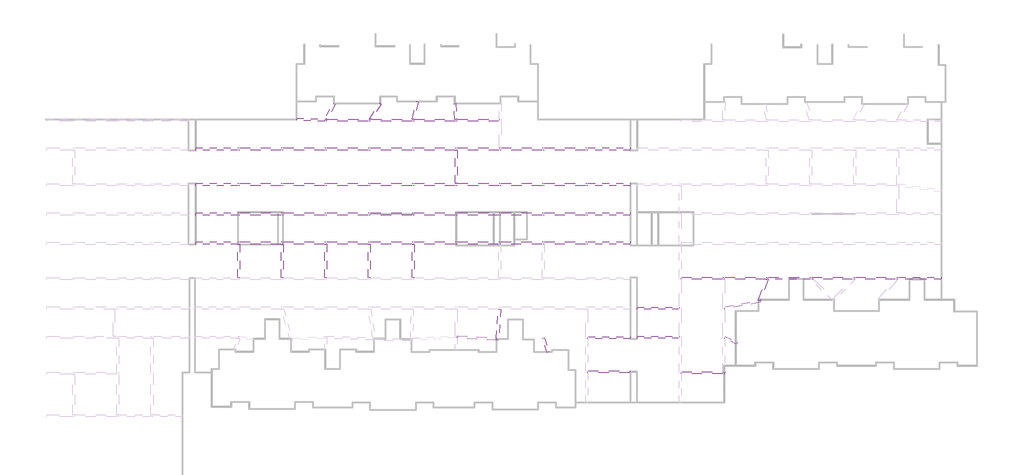
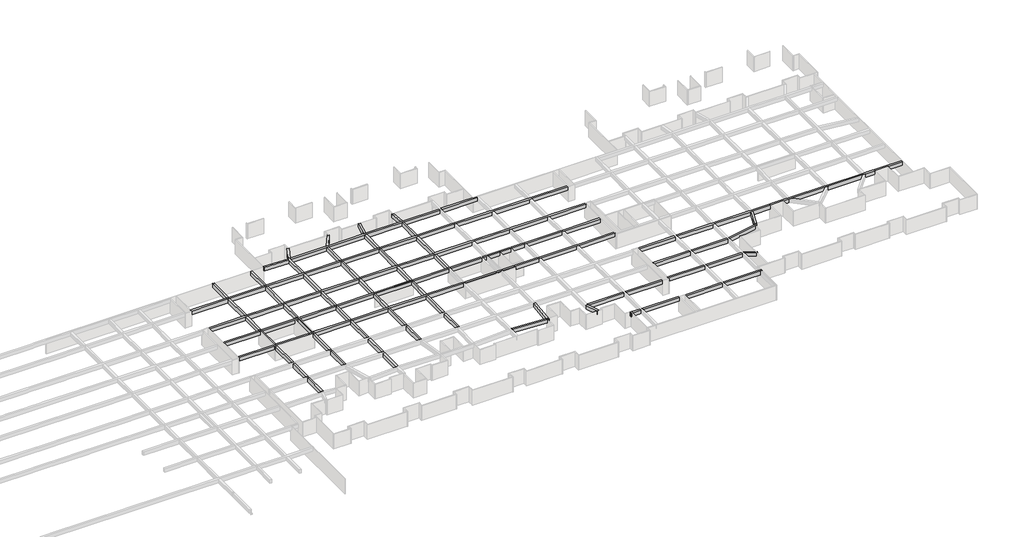
# One storey, part 15 of 16: 28 beams.
"""IFC4 building model written with IfcOpenShell, lengths in millimetres."""

from ifc_helpers import new_model, si_unit, frame, origin, place, context, project, spatial, polyline, outline, extrude, faceted_brep, element, save

model = new_model("IFC4")

# Units and contexts
model_context = context("Model", 3, world=origin())
ifc_project = project(units=[si_unit("LENGTHUNIT", "METRE", prefix="MILLI")], contexts=[model_context])

# Site, building, storey
site = spatial("IfcSite", under=ifc_project)
building = spatial("IfcBuilding", under=site)
storey = spatial("IfcBuildingStorey", under=building, Name="户型图", Elevation=0.0)

# Beams
placement = place(None, origin())
element("IfcBeam", 1, ObjectType="混凝土 - 矩形梁 : KL_beam", at=placement, inside=storey, context=model_context, shape_type="Brep", body=[
    faceted_brep([(413278.7576761, -137565.7214763, 3300.0), (413278.7576761, -137965.7214763, 3300.0), (413278.7576761, -137965.7214763, 2500.0), (413278.7576761, -137565.7214763, 2500.0), (333303.7576761, -137565.7214763, 3300.0), (333303.7576761, -137565.7214763, 2500.0), (333303.7576761, -137965.7214763, 2500.0), (333303.7576761, -137965.7214763, 3300.0), (405478.7576761, -137565.7214763, 3300.0), (405078.7576761, -137565.7214763, 3300.0), (397425.7298502, -137565.7214763, 3300.0), (397025.7298502, -137565.7214763, 3300.0), (389513.757676, -137565.7214763, 3300.0), (389113.757676, -137565.7214763, 3300.0), (381435.9353884, -137565.7214763, 3300.0), (381035.9353884, -137565.7214763, 3300.0), (373507.5350349, -137565.7214763, 3300.0), (373107.5350349, -137565.7214763, 3300.0), (365445.2144882, -137565.7214763, 3300.0), (365045.2144882, -137565.7214763, 3300.0), (357429.5901603, -137565.7214763, 3300.0), (357029.5901603, -137565.7214763, 3300.0), (349446.5285699, -137565.7214763, 3300.0), (349046.5285699, -137565.7214763, 3300.0), (341453.7576761, -137565.7214763, 3300.0), (341053.7576761, -137565.7214763, 3300.0), (341053.7576761, -137965.7214763, 3300.0), (341453.7576761, -137965.7214763, 3300.0), (349046.5285699, -137965.7214763, 3300.0), (349446.5285699, -137965.7214763, 3300.0), (357029.5901603, -137965.7214763, 3300.0), (357429.5901603, -137965.7214763, 3300.0), (365045.2144882, -137965.7214763, 3300.0), (365445.2144882, -137965.7214763, 3300.0), (373107.5350349, -137965.7214763, 3300.0), (373507.5350349, -137965.7214763, 3300.0), (381035.9353884, -137965.7214763, 3300.0), (381435.9353884, -137965.7214763, 3300.0), (389113.757676, -137965.7214763, 3300.0), (389513.757676, -137965.7214763, 3300.0), (397025.7298502, -137965.7214763, 3300.0), (397425.7298502, -137965.7214763, 3300.0), (405078.7576761, -137965.7214763, 3300.0), (405478.7576761, -137965.7214763, 3300.0), (341053.7576761, -137965.7214763, 2500.0), (341453.7576761, -137965.7214763, 2500.0), (349046.5285699, -137965.7214763, 2500.0), (349446.5285699, -137965.7214763, 2500.0), (357029.5901603, -137965.7214763, 2500.0), (357429.5901603, -137965.7214763, 2500.0), (365045.2144882, -137965.7214763, 2500.0), (365445.2144882, -137965.7214763, 2500.0), (373107.5350349, -137965.7214763, 2500.0), (373507.5350349, -137965.7214763, 2500.0), (381035.9353884, -137965.7214763, 2500.0), (381435.9353884, -137965.7214763, 2500.0), (389113.757676, -137965.7214763, 2500.0), (389513.757676, -137965.7214763, 2500.0), (397025.7298502, -137965.7214763, 2500.0), (397425.7298502, -137965.7214763, 2500.0), (405078.7576761, -137965.7214763, 2500.0), (405478.7576761, -137965.7214763, 2500.0), (341053.7576761, -137565.7214763, 2500.0), (341453.7576761, -137565.7214763, 2500.0), (349046.5285699, -137565.7214763, 2500.0), (349446.5285699, -137565.7214763, 2500.0), (357029.5901603, -137565.7214763, 2500.0), (357429.5901603, -137565.7214763, 2500.0), (365045.2144882, -137565.7214763, 2500.0), (365445.2144882, -137565.7214763, 2500.0), (373107.5350349, -137565.7214763, 2500.0), (373507.5350349, -137565.7214763, 2500.0), (381035.9353884, -137565.7214763, 2500.0), (381435.9353884, -137565.7214763, 2500.0), (389113.757676, -137565.7214763, 2500.0), (389513.757676, -137565.7214763, 2500.0), (397025.7298502, -137565.7214763, 2500.0), (397425.7298502, -137565.7214763, 2500.0), (405078.7576761, -137565.7214763, 2500.0), (405478.7576761, -137565.7214763, 2500.0)], [[[0, 1, 2, 3]], [[4, 5, 6, 7]], [[1, 0, 8, 9, 10, 11, 12, 13, 14, 15, 16, 17, 18, 19, 20, 21, 22, 23, 24, 25, 4, 7, 26, 27, 28, 29, 30, 31, 32, 33, 34, 35, 36, 37, 38, 39, 40, 41, 42, 43]], [[2, 1, 43, 42, 41, 40, 39, 38, 37, 36, 35, 34, 33, 32, 31, 30, 29, 28, 27, 26, 7, 6, 44, 45, 46, 47, 48, 49, 50, 51, 52, 53, 54, 55, 56, 57, 58, 59, 60, 61]], [[3, 2, 61, 60, 59, 58, 57, 56, 55, 54, 53, 52, 51, 50, 49, 48, 47, 46, 45, 44, 6, 5, 62, 63, 64, 65, 66, 67, 68, 69, 70, 71, 72, 73, 74, 75, 76, 77, 78, 79]], [[0, 3, 79, 78, 77, 76, 75, 74, 73, 72, 71, 70, 69, 68, 67, 66, 65, 64, 63, 62, 5, 4, 25, 24, 23, 22, 21, 20, 19, 18, 17, 16, 15, 14, 13, 12, 11, 10, 9, 8]]]),
])
element("IfcBeam", 2, ObjectType="混凝土 - 矩形梁 : KL_beam", at=placement, inside=storey, context=model_context, shape_type="Brep", body=[
    faceted_brep([(413278.7576761, -144085.7214763, 3300.0), (413278.7576761, -144485.7214763, 3300.0), (413278.7576761, -144485.7214763, 2500.0), (413278.7576761, -144085.7214763, 2500.0), (333303.7576761, -144085.7214763, 3300.0), (333303.7576761, -144085.7214763, 2500.0), (333303.7576761, -144485.7214763, 2500.0), (333303.7576761, -144485.7214763, 3300.0), (405478.7576761, -144085.7214763, 3300.0), (405078.7576761, -144085.7214763, 3300.0), (397425.7298502, -144085.7214763, 3300.0), (397025.7298502, -144085.7214763, 3300.0), (389513.757676, -144085.7214763, 3300.0), (389113.757676, -144085.7214763, 3300.0), (381435.9353884, -144085.7214763, 3300.0), (381035.9353884, -144085.7214763, 3300.0), (373507.5350349, -144085.7214763, 3300.0), (373107.5350349, -144085.7214763, 3300.0), (365445.2144882, -144085.7214763, 3300.0), (365045.2144882, -144085.7214763, 3300.0), (357429.5901603, -144085.7214763, 3300.0), (357029.5901603, -144085.7214763, 3300.0), (349446.5285699, -144085.7214763, 3300.0), (349046.5285699, -144085.7214763, 3300.0), (341453.7576761, -144085.7214763, 3300.0), (341053.7576761, -144085.7214763, 3300.0), (341053.7576761, -144485.7214763, 3300.0), (341453.7576761, -144485.7214763, 3300.0), (349046.5285699, -144485.7214763, 3300.0), (349446.5285699, -144485.7214763, 3300.0), (357029.5901603, -144485.7214763, 3300.0), (357429.5901603, -144485.7214763, 3300.0), (365045.2144882, -144485.7214763, 3300.0), (365445.2144882, -144485.7214763, 3300.0), (373107.5350349, -144485.7214763, 3300.0), (373507.5350349, -144485.7214763, 3300.0), (381035.9353884, -144485.7214763, 3300.0), (381435.9353884, -144485.7214763, 3300.0), (389113.757676, -144485.7214763, 3300.0), (389513.757676, -144485.7214763, 3300.0), (397025.7298502, -144485.7214763, 3300.0), (397425.7298502, -144485.7214763, 3300.0), (405078.7576761, -144485.7214763, 3300.0), (405478.7576761, -144485.7214763, 3300.0), (341053.7576761, -144485.7214763, 2500.0), (341453.7576761, -144485.7214763, 2500.0), (349046.5285699, -144485.7214763, 2500.0), (349446.5285699, -144485.7214763, 2500.0), (357029.5901603, -144485.7214763, 2500.0), (357429.5901603, -144485.7214763, 2500.0), (365045.2144882, -144485.7214763, 2500.0), (365445.2144882, -144485.7214763, 2500.0), (373107.5350349, -144485.7214763, 2500.0), (373507.5350349, -144485.7214763, 2500.0), (381035.9353884, -144485.7214763, 2500.0), (381435.9353884, -144485.7214763, 2500.0), (389113.757676, -144485.7214763, 2500.0), (389513.757676, -144485.7214763, 2500.0), (397025.7298502, -144485.7214763, 2500.0), (397425.7298502, -144485.7214763, 2500.0), (405078.7576761, -144485.7214763, 2500.0), (405478.7576761, -144485.7214763, 2500.0), (341053.7576761, -144085.7214763, 2500.0), (341453.7576761, -144085.7214763, 2500.0), (349046.5285699, -144085.7214763, 2500.0), (349446.5285699, -144085.7214763, 2500.0), (357029.5901603, -144085.7214763, 2500.0), (357429.5901603, -144085.7214763, 2500.0), (365045.2144882, -144085.7214763, 2500.0), (365445.2144882, -144085.7214763, 2500.0), (373107.5350349, -144085.7214763, 2500.0), (373507.5350349, -144085.7214763, 2500.0), (381035.9353884, -144085.7214763, 2500.0), (381435.9353884, -144085.7214763, 2500.0), (389113.757676, -144085.7214763, 2500.0), (389513.757676, -144085.7214763, 2500.0), (397025.7298502, -144085.7214763, 2500.0), (397425.7298502, -144085.7214763, 2500.0), (405078.7576761, -144085.7214763, 2500.0), (405478.7576761, -144085.7214763, 2500.0)], [[[0, 1, 2, 3]], [[4, 5, 6, 7]], [[1, 0, 8, 9, 10, 11, 12, 13, 14, 15, 16, 17, 18, 19, 20, 21, 22, 23, 24, 25, 4, 7, 26, 27, 28, 29, 30, 31, 32, 33, 34, 35, 36, 37, 38, 39, 40, 41, 42, 43]], [[2, 1, 43, 42, 41, 40, 39, 38, 37, 36, 35, 34, 33, 32, 31, 30, 29, 28, 27, 26, 7, 6, 44, 45, 46, 47, 48, 49, 50, 51, 52, 53, 54, 55, 56, 57, 58, 59, 60, 61]], [[3, 2, 61, 60, 59, 58, 57, 56, 55, 54, 53, 52, 51, 50, 49, 48, 47, 46, 45, 44, 6, 5, 62, 63, 64, 65, 66, 67, 68, 69, 70, 71, 72, 73, 74, 75, 76, 77, 78, 79]], [[0, 3, 79, 78, 77, 76, 75, 74, 73, 72, 71, 70, 69, 68, 67, 66, 65, 64, 63, 62, 5, 4, 25, 24, 23, 22, 21, 20, 19, 18, 17, 16, 15, 14, 13, 12, 11, 10, 9, 8]]]),
])
element("IfcBeam", 3, ObjectType="混凝土 - 矩形梁 : KL_beam", at=placement, inside=storey, context=model_context, shape_type="Brep", body=[
    faceted_brep([(413278.7576761, -149515.4343269, 3300.0), (413278.7576761, -149915.4343269, 3300.0), (413278.7576761, -149915.4343269, 2500.0), (413278.7576761, -149515.4343269, 2500.0), (333303.7576761, -149515.4343269, 3300.0), (333303.7576761, -149515.4343269, 2500.0), (333303.7576761, -149915.4343269, 2500.0), (333303.7576761, -149915.4343269, 3300.0), (405478.7576761, -149515.4343269, 3300.0), (405078.7576761, -149515.4343269, 3300.0), (397425.7298502, -149515.4343269, 3300.0), (397025.7298502, -149515.4343269, 3300.0), (389513.757676, -149515.4343269, 3300.0), (389113.757676, -149515.4343269, 3300.0), (381435.9353884, -149515.4343269, 3300.0), (381035.9353884, -149515.4343269, 3300.0), (373507.5350349, -149515.4343269, 3300.0), (373107.5350349, -149515.4343269, 3300.0), (365445.2144882, -149515.4343269, 3300.0), (365045.2144882, -149515.4343269, 3300.0), (357429.5901603, -149515.4343269, 3300.0), (357029.5901603, -149515.4343269, 3300.0), (349446.5285699, -149515.4343269, 3300.0), (349046.5285699, -149515.4343269, 3300.0), (341453.7576761, -149515.4343269, 3300.0), (341053.7576761, -149515.4343269, 3300.0), (341053.7576761, -149915.4343269, 3300.0), (341453.7576761, -149915.4343269, 3300.0), (349046.5285699, -149915.4343269, 3300.0), (349446.5285699, -149915.4343269, 3300.0), (357029.5901603, -149915.4343269, 3300.0), (357429.5901603, -149915.4343269, 3300.0), (365045.2144882, -149915.4343269, 3300.0), (365445.2144882, -149915.4343269, 3300.0), (373107.5350349, -149915.4343269, 3300.0), (373507.5350349, -149915.4343269, 3300.0), (381035.9353884, -149915.4343269, 3300.0), (381435.9353884, -149915.4343269, 3300.0), (389033.5747738, -149915.4343269, 3300.0), (389433.5747738, -149915.4343269, 3300.0), (397025.7298502, -149915.4343269, 3300.0), (397425.7298502, -149915.4343269, 3300.0), (405078.7576761, -149915.4343269, 3300.0), (405478.7576761, -149915.4343269, 3300.0), (341053.7576761, -149915.4343269, 2500.0), (341453.7576761, -149915.4343269, 2500.0), (349046.5285699, -149915.4343269, 2500.0), (349446.5285699, -149915.4343269, 2500.0), (357029.5901603, -149915.4343269, 2500.0), (357429.5901603, -149915.4343269, 2500.0), (365045.2144882, -149915.4343269, 2500.0), (365445.2144882, -149915.4343269, 2500.0), (373107.5350349, -149915.4343269, 2500.0), (373507.5350349, -149915.4343269, 2500.0), (381035.9353884, -149915.4343269, 2500.0), (381435.9353884, -149915.4343269, 2500.0), (389033.5747738, -149915.4343269, 2500.0), (389433.5747738, -149915.4343269, 2500.0), (397025.7298502, -149915.4343269, 2500.0), (397425.7298502, -149915.4343269, 2500.0), (405078.7576761, -149915.4343269, 2500.0), (405478.7576761, -149915.4343269, 2500.0), (341053.7576761, -149515.4343269, 2500.0), (341453.7576761, -149515.4343269, 2500.0), (349046.5285699, -149515.4343269, 2500.0), (349446.5285699, -149515.4343269, 2500.0), (357029.5901603, -149515.4343269, 2500.0), (357429.5901603, -149515.4343269, 2500.0), (365045.2144882, -149515.4343269, 2500.0), (365445.2144882, -149515.4343269, 2500.0), (373107.5350349, -149515.4343269, 2500.0), (373507.5350349, -149515.4343269, 2500.0), (381035.9353884, -149515.4343269, 2500.0), (381435.9353884, -149515.4343269, 2500.0), (389113.757676, -149515.4343269, 2500.0), (389513.757676, -149515.4343269, 2500.0), (397025.7298502, -149515.4343269, 2500.0), (397425.7298502, -149515.4343269, 2500.0), (405078.7576761, -149515.4343269, 2500.0), (405478.7576761, -149515.4343269, 2500.0)], [[[0, 1, 2, 3]], [[4, 5, 6, 7]], [[1, 0, 8, 9, 10, 11, 12, 13, 14, 15, 16, 17, 18, 19, 20, 21, 22, 23, 24, 25, 4, 7, 26, 27, 28, 29, 30, 31, 32, 33, 34, 35, 36, 37, 38, 39, 40, 41, 42, 43]], [[2, 1, 43, 42, 41, 40, 39, 38, 37, 36, 35, 34, 33, 32, 31, 30, 29, 28, 27, 26, 7, 6, 44, 45, 46, 47, 48, 49, 50, 51, 52, 53, 54, 55, 56, 57, 58, 59, 60, 61]], [[3, 2, 61, 60, 59, 58, 57, 56, 55, 54, 53, 52, 51, 50, 49, 48, 47, 46, 45, 44, 6, 5, 62, 63, 64, 65, 66, 67, 68, 69, 70, 71, 72, 73, 74, 75, 76, 77, 78, 79]], [[0, 3, 79, 78, 77, 76, 75, 74, 73, 72, 71, 70, 69, 68, 67, 66, 65, 64, 63, 62, 5, 4, 25, 24, 23, 22, 21, 20, 19, 18, 17, 16, 15, 14, 13, 12, 11, 10, 9, 8]]]),
])
element("IfcBeam", 4, ObjectType="混凝土 - 矩形梁 : KL_beam", at=placement, inside=storey, context=model_context, shape_type="Brep", body=[
    faceted_brep([(413278.7576761, -154845.1471774, 3300.0), (413278.7576761, -155245.1471774, 3300.0), (413278.7576761, -155245.1471774, 2500.0), (413278.7576761, -154845.1471774, 2500.0), (333303.7576761, -154845.1471774, 3300.0), (333303.7576761, -154845.1471774, 2500.0), (333303.7576761, -155245.1471774, 2500.0), (333303.7576761, -155245.1471774, 3300.0), (405478.7576761, -154845.1471774, 3300.0), (405078.7576761, -154845.1471774, 3300.0), (397425.7298502, -154845.1471774, 3300.0), (397025.7298502, -154845.1471774, 3300.0), (389433.5747738, -154845.1471774, 3300.0), (389033.5747738, -154845.1471774, 3300.0), (381435.9353884, -154845.1471774, 3300.0), (381035.9353884, -154845.1471774, 3300.0), (373507.5350349, -154845.1471774, 3300.0), (373107.5350349, -154845.1471774, 3300.0), (365445.2144882, -154845.1471774, 3300.0), (365045.2144882, -154845.1471774, 3300.0), (357429.5901603, -154845.1471774, 3300.0), (357029.5901603, -154845.1471774, 3300.0), (349446.5285699, -154845.1471774, 3300.0), (349046.5285699, -154845.1471774, 3300.0), (341453.7576761, -154845.1471774, 3300.0), (341053.7576761, -154845.1471774, 3300.0), (341053.7576761, -155245.1471774, 3300.0), (341453.7576761, -155245.1471774, 3300.0), (349046.5285699, -155245.1471774, 3300.0), (349446.5285699, -155245.1471774, 3300.0), (357029.5901603, -155245.1471774, 3300.0), (357429.5901603, -155245.1471774, 3300.0), (365045.2144882, -155245.1471774, 3300.0), (365445.2144882, -155245.1471774, 3300.0), (373107.5350349, -155245.1471774, 3300.0), (373507.5350349, -155245.1471774, 3300.0), (381035.9353884, -155245.1471774, 3300.0), (381435.9353884, -155245.1471774, 3300.0), (389033.5747738, -155245.1471774, 3300.0), (389433.5747738, -155245.1471774, 3300.0), (397025.7298502, -155245.1471774, 3300.0), (397425.7298502, -155245.1471774, 3300.0), (405078.7576761, -155245.1471774, 3300.0), (405478.7576761, -155245.1471774, 3300.0), (341053.7576761, -155245.1471774, 2500.0), (341453.7576761, -155245.1471774, 2500.0), (349046.5285699, -155245.1471774, 2500.0), (349446.5285699, -155245.1471774, 2500.0), (357029.5901603, -155245.1471774, 2500.0), (357429.5901603, -155245.1471774, 2500.0), (365045.2144882, -155245.1471774, 2500.0), (365445.2144882, -155245.1471774, 2500.0), (373107.5350349, -155245.1471774, 2500.0), (373507.5350349, -155245.1471774, 2500.0), (381035.9353884, -155245.1471774, 2500.0), (381435.9353884, -155245.1471774, 2500.0), (389033.5747738, -155245.1471774, 2500.0), (389433.5747738, -155245.1471774, 2500.0), (397025.7298502, -155245.1471774, 2500.0), (397425.7298502, -155245.1471774, 2500.0), (405078.7576761, -155245.1471774, 2500.0), (405478.7576761, -155245.1471774, 2500.0), (341053.7576761, -154845.1471774, 2500.0), (341453.7576761, -154845.1471774, 2500.0), (349046.5285699, -154845.1471774, 2500.0), (349446.5285699, -154845.1471774, 2500.0), (357029.5901603, -154845.1471774, 2500.0), (357429.5901603, -154845.1471774, 2500.0), (365045.2144882, -154845.1471774, 2500.0), (365445.2144882, -154845.1471774, 2500.0), (373107.5350349, -154845.1471774, 2500.0), (373507.5350349, -154845.1471774, 2500.0), (381035.9353884, -154845.1471774, 2500.0), (381435.9353884, -154845.1471774, 2500.0), (389033.5747738, -154845.1471774, 2500.0), (389433.5747738, -154845.1471774, 2500.0), (397025.7298502, -154845.1471774, 2500.0), (397425.7298502, -154845.1471774, 2500.0), (405078.7576761, -154845.1471774, 2500.0), (405478.7576761, -154845.1471774, 2500.0)], [[[0, 1, 2, 3]], [[4, 5, 6, 7]], [[1, 0, 8, 9, 10, 11, 12, 13, 14, 15, 16, 17, 18, 19, 20, 21, 22, 23, 24, 25, 4, 7, 26, 27, 28, 29, 30, 31, 32, 33, 34, 35, 36, 37, 38, 39, 40, 41, 42, 43]], [[2, 1, 43, 42, 41, 40, 39, 38, 37, 36, 35, 34, 33, 32, 31, 30, 29, 28, 27, 26, 7, 6, 44, 45, 46, 47, 48, 49, 50, 51, 52, 53, 54, 55, 56, 57, 58, 59, 60, 61]], [[3, 2, 61, 60, 59, 58, 57, 56, 55, 54, 53, 52, 51, 50, 49, 48, 47, 46, 45, 44, 6, 5, 62, 63, 64, 65, 66, 67, 68, 69, 70, 71, 72, 73, 74, 75, 76, 77, 78, 79]], [[0, 3, 79, 78, 77, 76, 75, 74, 73, 72, 71, 70, 69, 68, 67, 66, 65, 64, 63, 62, 5, 4, 25, 24, 23, 22, 21, 20, 19, 18, 17, 16, 15, 14, 13, 12, 11, 10, 9, 8]]]),
])
element("IfcBeam", 5, ObjectType="混凝土 - 矩形梁 : KL_beam", at=placement, inside=storey, context=model_context, shape_type="Brep", body=[
    faceted_brep([(341053.7576761, -132205.3490877, 3300.0), (341453.7576761, -132205.3490877, 3300.0), (341453.7576761, -132205.3490877, 2500.0), (341053.7576761, -132205.3490877, 2500.0), (341053.7576761, -137565.7214763, 3300.0), (341453.7576761, -137565.7214763, 3300.0), (341453.7576761, -137565.7214763, 2500.0), (341053.7576761, -137565.7214763, 2500.0)], [[[0, 1, 2, 3]], [[1, 0, 4, 5]], [[2, 1, 5, 6]], [[3, 2, 6, 7]], [[0, 3, 7, 4]], [[5, 4, 7, 6]]]),
    faceted_brep([(341053.7576761, -172220.550998, 3300.0), (341053.7576761, -172220.550998, 2500.0), (341105.8656487, -172220.550998, 2500.0), (341263.4411641, -172220.550998, 2500.0), (341263.4411641, -172220.550998, 3300.0), (341105.8656487, -172220.550998, 3300.0), (341453.7576761, -172239.0235791, 3300.0), (341453.7576761, -172239.0235791, 2500.0), (341053.7576761, -167205.1471774, 3300.0), (341453.7576761, -167205.1471774, 3300.0), (341453.7576761, -167205.1471774, 2500.0), (341053.7576761, -167205.1471774, 2500.0)], [[[0, 1, 2, 3, 4, 5]], [[6, 4, 3, 7]], [[8, 9, 10, 11]], [[4, 6, 9, 8, 0, 5]], [[6, 7, 10, 9]], [[7, 3, 2, 1, 11, 10]], [[1, 0, 8, 11]]]),
    faceted_brep([(341053.7576761, -137965.7214763, 3300.0), (341453.7576761, -137965.7214763, 3300.0), (341453.7576761, -137965.7214763, 2500.0), (341053.7576761, -137965.7214763, 2500.0), (341053.7576761, -144085.7214763, 3300.0), (341453.7576761, -144085.7214763, 3300.0), (341453.7576761, -144085.7214763, 2500.0), (341053.7576761, -144085.7214763, 2500.0)], [[[0, 1, 2, 3]], [[1, 0, 4, 5]], [[2, 1, 5, 6]], [[3, 2, 6, 7]], [[0, 3, 7, 4]], [[5, 4, 7, 6]]]),
    faceted_brep([(341053.7576761, -144485.7214763, 3300.0), (341453.7576761, -144485.7214763, 3300.0), (341453.7576761, -144485.7214763, 2500.0), (341053.7576761, -144485.7214763, 2500.0), (341053.7576761, -149515.4343269, 3300.0), (341453.7576761, -149515.4343269, 3300.0), (341453.7576761, -149515.4343269, 2500.0), (341053.7576761, -149515.4343269, 2500.0)], [[[0, 1, 2, 3]], [[1, 0, 4, 5]], [[2, 1, 5, 6]], [[3, 2, 6, 7]], [[0, 3, 7, 4]], [[5, 4, 7, 6]]]),
    faceted_brep([(341053.7576761, -149915.4343269, 3300.0), (341453.7576761, -149915.4343269, 3300.0), (341453.7576761, -149915.4343269, 2500.0), (341053.7576761, -149915.4343269, 2500.0), (341053.7576761, -154845.1471774, 3300.0), (341453.7576761, -154845.1471774, 3300.0), (341453.7576761, -154845.1471774, 2500.0), (341053.7576761, -154845.1471774, 2500.0)], [[[0, 1, 2, 3]], [[1, 0, 4, 5]], [[2, 1, 5, 6]], [[3, 2, 6, 7]], [[0, 3, 7, 4]], [[5, 4, 7, 6]]]),
    faceted_brep([(341053.7576761, -155245.1471774, 3300.0), (341453.7576761, -155245.1471774, 3300.0), (341453.7576761, -155245.1471774, 2500.0), (341053.7576761, -155245.1471774, 2500.0), (341053.7576761, -161426.0461868, 3300.0), (341453.7576761, -161426.0461868, 3300.0), (341453.7576761, -161426.0461868, 2500.0), (341053.7576761, -161426.0461868, 2500.0)], [[[0, 1, 2, 3]], [[1, 0, 4, 5]], [[2, 1, 5, 6]], [[3, 2, 6, 7]], [[0, 3, 7, 4]], [[5, 4, 7, 6]]]),
    faceted_brep([(341053.7576761, -161826.0461868, 3300.0), (341453.7576761, -161826.0461868, 3300.0), (341453.7576761, -161826.0461868, 2500.0), (341053.7576761, -161826.0461868, 2500.0), (341053.7576761, -166805.1471774, 3300.0), (341453.7576761, -166805.1471774, 3300.0), (341453.7576761, -166805.1471774, 2500.0), (341053.7576761, -166805.1471774, 2500.0)], [[[0, 1, 2, 3]], [[1, 0, 4, 5]], [[2, 1, 5, 6]], [[3, 2, 6, 7]], [[0, 3, 7, 4]], [[5, 4, 7, 6]]]),
])
element("IfcBeam", 6, ObjectType="混凝土 - 矩形梁 : KL_beam", at=placement, inside=storey, context=model_context, shape_type="SweptSolid", body=[
    extrude(outline(polyline([(349046.5285699, -132305.1471774), (349446.5285699, -132305.1471774), (349446.5285699, -137565.7214763), (349046.5285699, -137565.7214763), (349046.5285699, -132305.1471774)])), frame((0.0, 0.0, 2500.0), z_axis=(0.0, 0.0, 1.0), x_axis=(1.0, 0.0, 0.0)), (0.0, 0.0, 1.0), 800.0),
    extrude(outline(polyline([(349046.5285699, -137965.7214763), (349446.5285699, -137965.7214763), (349446.5285699, -144085.7214763), (349046.5285699, -144085.7214763), (349046.5285699, -137965.7214763)])), frame((0.0, 0.0, 2500.0), z_axis=(0.0, 0.0, 1.0), x_axis=(1.0, 0.0, 0.0)), (0.0, 0.0, 1.0), 800.0),
    extrude(outline(polyline([(349446.5285699, -166805.1471774), (349046.5285699, -166805.1471774), (349046.5285699, -161826.0461868), (349446.5285699, -161826.0461868), (349446.5285699, -166805.1471774)])), frame((0.0, 0.0, 2500.0), z_axis=(0.0, 0.0, 1.0), x_axis=(1.0, 0.0, 0.0)), (0.0, 0.0, 1.0), 800.0),
    extrude(outline(polyline([(349046.5285699, -144485.7214763), (349446.5285699, -144485.7214763), (349446.5285699, -149515.4343269), (349046.5285699, -149515.4343269), (349046.5285699, -144485.7214763)])), frame((0.0, 0.0, 2500.0), z_axis=(0.0, 0.0, 1.0), x_axis=(1.0, 0.0, 0.0)), (0.0, 0.0, 1.0), 800.0),
    extrude(outline(polyline([(349046.5285699, -149915.4343269), (349446.5285699, -149915.4343269), (349446.5285699, -154845.1471774), (349046.5285699, -154845.1471774), (349046.5285699, -149915.4343269)])), frame((0.0, 0.0, 2500.0), z_axis=(0.0, 0.0, 1.0), x_axis=(1.0, 0.0, 0.0)), (0.0, 0.0, 1.0), 800.0),
    extrude(outline(polyline([(349046.5285699, -155245.1471774), (349446.5285699, -155245.1471774), (349446.5285699, -161426.0461868), (349046.5285699, -161426.0461868), (349046.5285699, -155245.1471774)])), frame((0.0, 0.0, 2500.0), z_axis=(0.0, 0.0, 1.0), x_axis=(1.0, 0.0, 0.0)), (0.0, 0.0, 1.0), 800.0),
])
element("IfcBeam", 7, ObjectType="混凝土 - 矩形梁 : KL_beam", at=placement, inside=storey, context=model_context, shape_type="Brep", body=[
    faceted_brep([(357029.5901603, -137565.7214763, 3300.0), (357429.5901603, -137565.7214763, 3300.0), (357429.5901603, -132682.1518701, 3300.0), (357429.5901603, -132528.9518593, 3300.0), (357429.5901603, -131627.4508185, 3300.0), (357107.4901686, -132278.0131322, 3300.0), (357029.5901603, -132435.3518808, 3300.0), (357029.5901603, -132675.6598872, 3300.0), (357429.5901603, -137565.7214763, 2500.0), (357429.5901603, -132682.1518701, 2500.0), (357429.5901603, -132528.9518593, 2500.0), (357429.5901603, -131627.4508185, 2500.0), (357029.5901603, -137565.7214763, 2500.0), (357029.5901603, -132675.6598872, 2500.0), (357029.5901603, -132435.3518808, 2500.0), (357107.4901686, -132278.0131322, 2500.0)], [[[0, 1, 2, 3, 4, 5, 6, 7]], [[1, 8, 9, 10, 11, 4, 3, 2]], [[8, 12, 13, 14, 15, 11, 10, 9]], [[12, 0, 7, 6, 14, 13]], [[1, 0, 12, 8]], [[6, 5, 4, 11, 15, 14]]]),
    faceted_brep([(357029.5901603, -137965.7214763, 3300.0), (357429.5901603, -137965.7214763, 3300.0), (357429.5901603, -137965.7214763, 2500.0), (357029.5901603, -137965.7214763, 2500.0), (357029.5901603, -144085.7214763, 3300.0), (357429.5901603, -144085.7214763, 3300.0), (357429.5901603, -144085.7214763, 2500.0), (357029.5901603, -144085.7214763, 2500.0)], [[[0, 1, 2, 3]], [[1, 0, 4, 5]], [[2, 1, 5, 6]], [[3, 2, 6, 7]], [[0, 3, 7, 4]], [[5, 4, 7, 6]]]),
    faceted_brep([(357029.5901603, -144485.7214763, 3300.0), (357429.5901603, -144485.7214763, 3300.0), (357429.5901603, -144485.7214763, 2500.0), (357029.5901603, -144485.7214763, 2500.0), (357029.5901603, -149515.4343269, 3300.0), (357429.5901603, -149515.4343269, 3300.0), (357429.5901603, -149515.4343269, 2500.0), (357029.5901603, -149515.4343269, 2500.0)], [[[0, 1, 2, 3]], [[1, 0, 4, 5]], [[2, 1, 5, 6]], [[3, 2, 6, 7]], [[0, 3, 7, 4]], [[5, 4, 7, 6]]]),
    faceted_brep([(357029.5901603, -149915.4343269, 3300.0), (357429.5901603, -149915.4343269, 3300.0), (357429.5901603, -149915.4343269, 2500.0), (357029.5901603, -149915.4343269, 2500.0), (357029.5901603, -154845.1471774, 3300.0), (357429.5901603, -154845.1471774, 3300.0), (357429.5901603, -154845.1471774, 2500.0), (357029.5901603, -154845.1471774, 2500.0)], [[[0, 1, 2, 3]], [[1, 0, 4, 5]], [[2, 1, 5, 6]], [[3, 2, 6, 7]], [[0, 3, 7, 4]], [[5, 4, 7, 6]]]),
    faceted_brep([(357029.5901603, -155245.1471774, 3300.0), (357429.5901603, -155245.1471774, 3300.0), (357429.5901603, -155245.1471774, 2500.0), (357029.5901603, -155245.1471774, 2500.0), (357029.5901603, -161426.0461868, 3300.0), (357429.5901603, -161426.0461868, 3300.0), (357429.5901603, -161426.0461868, 2500.0), (357029.5901603, -161426.0461868, 2500.0)], [[[0, 1, 2, 3]], [[1, 0, 4, 5]], [[2, 1, 5, 6]], [[3, 2, 6, 7]], [[0, 3, 7, 4]], [[5, 4, 7, 6]]]),
    faceted_brep([(357029.5901603, -161826.0461868, 3300.0), (357429.5901603, -161826.0461868, 3300.0), (357429.5901603, -161826.0461868, 2500.0), (357029.5901603, -161826.0461868, 2500.0), (357029.5901603, -166805.1471774, 3300.0), (357429.5901603, -166805.1471774, 3300.0), (357429.5901603, -166805.1471774, 2500.0), (357029.5901603, -166805.1471774, 2500.0)], [[[0, 1, 2, 3]], [[1, 0, 4, 5]], [[2, 1, 5, 6]], [[3, 2, 6, 7]], [[0, 3, 7, 4]], [[5, 4, 7, 6]]]),
    faceted_brep([(357029.5901603, -167205.1471774, 3300.0), (357429.5901603, -167205.1471774, 3300.0), (357429.5901603, -167205.1471774, 2500.0), (357029.5901603, -167205.1471774, 2500.0), (357029.5901603, -172194.5475715, 3300.0), (357429.5901603, -172168.9371393, 3300.0), (357429.5901603, -172168.9371393, 2500.0), (357029.5901603, -172194.5475715, 2500.0)], [[[0, 1, 2, 3]], [[1, 0, 4, 5]], [[2, 1, 5, 6]], [[3, 2, 6, 7]], [[0, 3, 7, 4]], [[5, 4, 7, 6]]]),
])
element("IfcBeam", 8, ObjectType="混凝土 - 矩形梁 : KL_beam", at=placement, inside=storey, context=model_context, shape_type="Brep", body=[
    faceted_brep([(358578.5409484, -129306.8544128, 3300.0), (358937.0102239, -129484.3361824, 3300.0), (358937.0102239, -129484.3361824, 2500.0), (358578.5409484, -129306.8544128, 2500.0), (357429.5901603, -131627.4508185, 3300.0), (357429.5901603, -132528.9518593, 3300.0), (357551.7833351, -132282.1518701, 3300.0), (357429.5901603, -132528.9518593, 2500.0), (357551.7833351, -132282.1518701, 2500.0), (357429.5901603, -131627.4508185, 2500.0)], [[[0, 1, 2, 3]], [[1, 0, 4, 5, 6]], [[2, 1, 6, 5, 7, 8]], [[3, 2, 8, 7, 9]], [[0, 3, 9, 4]], [[5, 4, 9, 7]]]),
])
element("IfcBeam", 9, ObjectType="混凝土 - 矩形梁 : KL_beam", at=placement, inside=storey, context=model_context, shape_type="SweptSolid", body=[
    extrude(outline(polyline([(367089.0963461, -129289.7981648), (367428.3155846, -129501.7658705), (365690.937587, -132282.1518701), (365219.2662256, -132282.1518701), (367089.0963461, -129289.7981648)])), frame((0.0, 0.0, 2500.0), z_axis=(0.0, 0.0, 1.0), x_axis=(1.0, 0.0, 0.0)), (0.0, 0.0, 1.0), 800.0),
])
element("IfcBeam", 10, ObjectType="混凝土 - 矩形梁 : KL_beam", at=placement, inside=storey, context=model_context, shape_type="SweptSolid", body=[
    extrude(outline(polyline([(365045.2144882, -132682.1518701), (365445.2144882, -132682.1518701), (365445.2144882, -137565.7214763), (365045.2144882, -137565.7214763), (365045.2144882, -132682.1518701)])), frame((0.0, 0.0, 2500.0), z_axis=(0.0, 0.0, 1.0), x_axis=(1.0, 0.0, 0.0)), (0.0, 0.0, 1.0), 800.0),
    extrude(outline(polyline([(365445.2144882, -166805.1471774), (365045.2144882, -166805.1471774), (365045.2144882, -161826.0461868), (365445.2144882, -161826.0461868), (365445.2144882, -166805.1471774)])), frame((0.0, 0.0, 2500.0), z_axis=(0.0, 0.0, 1.0), x_axis=(1.0, 0.0, 0.0)), (0.0, 0.0, 1.0), 800.0),
    extrude(outline(polyline([(365045.2144882, -137965.7214763), (365445.2144882, -137965.7214763), (365445.2144882, -144085.7214763), (365045.2144882, -144085.7214763), (365045.2144882, -137965.7214763)])), frame((0.0, 0.0, 2500.0), z_axis=(0.0, 0.0, 1.0), x_axis=(1.0, 0.0, 0.0)), (0.0, 0.0, 1.0), 800.0),
    extrude(outline(polyline([(365045.2144882, -144485.7214763), (365445.2144882, -144485.7214763), (365445.2144882, -149515.4343269), (365045.2144882, -149515.4343269), (365045.2144882, -144485.7214763)])), frame((0.0, 0.0, 2500.0), z_axis=(0.0, 0.0, 1.0), x_axis=(1.0, 0.0, 0.0)), (0.0, 0.0, 1.0), 800.0),
    extrude(outline(polyline([(365045.2144882, -149915.4343269), (365445.2144882, -149915.4343269), (365445.2144882, -154845.1471774), (365045.2144882, -154845.1471774), (365045.2144882, -149915.4343269)])), frame((0.0, 0.0, 2500.0), z_axis=(0.0, 0.0, 1.0), x_axis=(1.0, 0.0, 0.0)), (0.0, 0.0, 1.0), 800.0),
    extrude(outline(polyline([(365045.2144882, -155245.1471774), (365445.2144882, -155245.1471774), (365445.2144882, -161426.0461868), (365045.2144882, -161426.0461868), (365045.2144882, -155245.1471774)])), frame((0.0, 0.0, 2500.0), z_axis=(0.0, 0.0, 1.0), x_axis=(1.0, 0.0, 0.0)), (0.0, 0.0, 1.0), 800.0),
])
element("IfcBeam", 11, ObjectType="混凝土 - 矩形梁 : KL_beam", at=placement, inside=storey, context=model_context, shape_type="SweptSolid", body=[
    extrude(outline(polyline([(373507.5350349, -166805.1471774), (373107.5350349, -166805.1471774), (373107.5350349, -161826.0461868), (373507.5350349, -161826.0461868), (373507.5350349, -166805.1471774)])), frame((0.0, 0.0, 2500.0), z_axis=(0.0, 0.0, 1.0), x_axis=(1.0, 0.0, 0.0)), (0.0, 0.0, 1.0), 800.0),
    extrude(outline(polyline([(373107.5350349, -137965.7214763), (373507.5350349, -137965.7214763), (373507.5350349, -144085.7214763), (373107.5350349, -144085.7214763), (373107.5350349, -137965.7214763)])), frame((0.0, 0.0, 2500.0), z_axis=(0.0, 0.0, 1.0), x_axis=(1.0, 0.0, 0.0)), (0.0, 0.0, 1.0), 800.0),
    extrude(outline(polyline([(373507.5350349, -137565.7214763), (373107.5350349, -137565.7214763), (373107.5350349, -132682.1518701), (373507.5350349, -132682.1518701), (373507.5350349, -137565.7214763)])), frame((0.0, 0.0, 2500.0), z_axis=(0.0, 0.0, 1.0), x_axis=(1.0, 0.0, 0.0)), (0.0, 0.0, 1.0), 800.0),
    extrude(outline(polyline([(373107.5350349, -144485.7214763), (373507.5350349, -144485.7214763), (373507.5350349, -149515.4343269), (373107.5350349, -149515.4343269), (373107.5350349, -144485.7214763)])), frame((0.0, 0.0, 2500.0), z_axis=(0.0, 0.0, 1.0), x_axis=(1.0, 0.0, 0.0)), (0.0, 0.0, 1.0), 800.0),
    extrude(outline(polyline([(373107.5350349, -149915.4343269), (373507.5350349, -149915.4343269), (373507.5350349, -154845.1471774), (373107.5350349, -154845.1471774), (373107.5350349, -149915.4343269)])), frame((0.0, 0.0, 2500.0), z_axis=(0.0, 0.0, 1.0), x_axis=(1.0, 0.0, 0.0)), (0.0, 0.0, 1.0), 800.0),
    extrude(outline(polyline([(373107.5350349, -155245.1471774), (373507.5350349, -155245.1471774), (373507.5350349, -161426.0461868), (373107.5350349, -161426.0461868), (373107.5350349, -155245.1471774)])), frame((0.0, 0.0, 2500.0), z_axis=(0.0, 0.0, 1.0), x_axis=(1.0, 0.0, 0.0)), (0.0, 0.0, 1.0), 800.0),
])
element("IfcBeam", 12, ObjectType="混凝土 - 矩形梁 : KL_beam", at=placement, inside=storey, context=model_context, shape_type="SweptSolid", body=[
    extrude(outline(polyline([(373860.3365631, -128942.4735942), (374251.5956034, -129025.6382705), (373559.4022696, -132282.1518701), (373150.4660317, -132282.1518701), (373860.3365631, -128942.4735942)])), frame((0.0, 0.0, 2500.0), z_axis=(0.0, 0.0, 1.0), x_axis=(1.0, 0.0, 0.0)), (0.0, 0.0, 1.0), 800.0),
])
element("IfcBeam", 13, ObjectType="混凝土 - 矩形梁 : KL_beam", at=placement, inside=storey, context=model_context, shape_type="SweptSolid", body=[
    extrude(outline(polyline([(380757.8191352, -129413.1310898), (381156.2970145, -129378.2687927), (381410.353864, -132282.1518701), (381008.8259289, -132282.1518701), (380757.8191352, -129413.1310898)])), frame((0.0, 0.0, 2500.0), z_axis=(0.0, 0.0, 1.0), x_axis=(1.0, 0.0, 0.0)), (0.0, 0.0, 1.0), 800.0),
])
element("IfcBeam", 14, ObjectType="混凝土 - 矩形梁 : KL_beam", at=placement, inside=storey, context=model_context, shape_type="SweptSolid", body=[
    extrude(outline(polyline([(381035.9353884, -132682.1518701), (381435.9353884, -132682.1518701), (381435.9353884, -137565.7214763), (381035.9353884, -137565.7214763), (381035.9353884, -132682.1518701)])), frame((0.0, 0.0, 2500.0), z_axis=(0.0, 0.0, 1.0), x_axis=(1.0, 0.0, 0.0)), (0.0, 0.0, 1.0), 800.0),
    extrude(outline(polyline([(381435.9353884, -149515.4343269), (381035.9353884, -149515.4343269), (381035.9353884, -144485.7214763), (381435.9353884, -144485.7214763), (381435.9353884, -149515.4343269)])), frame((0.0, 0.0, 2500.0), z_axis=(0.0, 0.0, 1.0), x_axis=(1.0, 0.0, 0.0)), (0.0, 0.0, 1.0), 800.0),
    extrude(outline(polyline([(381035.9353884, -137965.7214763), (381435.9353884, -137965.7214763), (381435.9353884, -144085.7214763), (381035.9353884, -144085.7214763), (381035.9353884, -137965.7214763)])), frame((0.0, 0.0, 2500.0), z_axis=(0.0, 0.0, 1.0), x_axis=(1.0, 0.0, 0.0)), (0.0, 0.0, 1.0), 800.0),
])
element("IfcBeam", 15, ObjectType="混凝土 - 矩形梁 : KL_beam", at=placement, inside=storey, context=model_context, shape_type="Brep", body=[
    faceted_brep([(398322.6513217, -175076.5277497, 3300.0), (397944.4438915, -175206.7550115, 3300.0), (397944.4438915, -175206.7550115, 2500.0), (398322.6513217, -175076.5277497, 2500.0), (397506.119509, -172705.1471775, 3300.0), (397425.7298502, -172471.6786556, 3300.0), (397025.7298502, -172538.6156993, 3300.0), (397025.7298502, -172538.6156993, 2500.0), (397425.7298502, -172471.6786556, 2500.0), (397506.119509, -172705.1471775, 2500.0)], [[[0, 1, 2, 3]], [[1, 0, 4, 5, 6]], [[2, 1, 6, 7]], [[3, 2, 7, 8, 9]], [[0, 3, 9, 8, 5, 4]], [[5, 8, 7, 6]]]),
])
element("IfcBeam", 16, ObjectType="混凝土 - 矩形梁 : KL_beam", at=placement, inside=storey, context=model_context, shape_type="Brep", body=[
    faceted_brep([(388618.1350696, -172939.2275831, 3300.0), (389017.4985034, -172962.2992125, 3300.0), (389420.0777911, -167205.1471774, 3300.0), (389019.1010318, -167205.1471774, 3300.0), (388646.039704, -172540.1727201, 3300.0), (389017.4985034, -172962.2992125, 2500.0), (389420.0777911, -167205.1471774, 2500.0), (388618.1350696, -172939.2275831, 2500.0), (388646.039704, -172540.1727201, 2500.0), (389019.1010318, -167205.1471774, 2500.0)], [[[0, 1, 2, 3, 4]], [[1, 5, 6, 2]], [[5, 7, 8, 9, 6]], [[7, 0, 4, 3, 9, 8]], [[3, 2, 6, 9]], [[1, 0, 7, 5]]]),
])
element("IfcBeam", 17, ObjectType="混凝土 - 矩形梁 : KL_beam", at=placement, inside=storey, context=model_context, shape_type="SweptSolid", body=[
    extrude(outline(polyline([(351860.4218943, -132505.0545297), (351873.6164745, -132105.2722101), (357107.4901686, -132278.0131322), (357029.5901603, -132435.3518808), (357029.5901603, -132675.6598872), (351860.4218943, -132505.0545297)])), frame((0.0, 0.0, 2500.0), z_axis=(0.0, 0.0, 1.0), x_axis=(1.0, 0.0, 0.0)), (0.0, 0.0, 1.0), 800.0),
])
element("IfcBeam", 18, ObjectType="混凝土 - 矩形梁 : KL_beam", at=placement, inside=storey, context=model_context, shape_type="Brep", body=[
    faceted_brep([(397025.7298502, -132682.1518701, 3300.0), (397025.7298502, -132282.1518701, 3300.0), (389513.757676, -132282.1518701, 3300.0), (389513.757676, -132682.1518701, 3300.0), (397025.7298502, -132682.1518701, 2500.0), (389513.757676, -132682.1518701, 2500.0), (397025.7298502, -132282.1518701, 2500.0), (389513.757676, -132282.1518701, 2500.0)], [[[0, 1, 2, 3]], [[4, 0, 3, 5]], [[6, 4, 5, 7]], [[1, 6, 7, 2]], [[1, 0, 4, 6]], [[3, 2, 7, 5]]]),
    faceted_brep([(357429.5901603, -132682.1518701, 2500.0), (357429.5901603, -132682.1518701, 3300.0), (357429.5901603, -132528.9518593, 3300.0), (357429.5901603, -132528.9518593, 2500.0), (357551.7833351, -132282.1518701, 3300.0), (357551.7833351, -132282.1518701, 2500.0), (357546.6561347, -132292.5075465, 2500.0), (357546.6561347, -132292.5075465, 3300.0), (389113.757676, -132282.1518701, 3300.0), (389113.757676, -132682.1518701, 3300.0), (389113.757676, -132682.1518701, 2500.0), (389113.757676, -132282.1518701, 2500.0), (365045.2144882, -132682.1518701, 3300.0), (365445.2144882, -132682.1518701, 3300.0), (373107.5350349, -132682.1518701, 3300.0), (373507.5350349, -132682.1518701, 3300.0), (381035.9353884, -132682.1518701, 3300.0), (381435.9353884, -132682.1518701, 3300.0), (381410.353864, -132282.1518701, 3300.0), (381008.8259289, -132282.1518701, 3300.0), (373559.4022696, -132282.1518701, 3300.0), (373150.4660317, -132282.1518701, 3300.0), (365690.937587, -132282.1518701, 3300.0), (365219.2662256, -132282.1518701, 3300.0), (365045.2144882, -132682.1518701, 2500.0), (365445.2144882, -132682.1518701, 2500.0), (373107.5350349, -132682.1518701, 2500.0), (373507.5350349, -132682.1518701, 2500.0), (381035.9353884, -132682.1518701, 2500.0), (381435.9353884, -132682.1518701, 2500.0), (365219.2662256, -132282.1518701, 2500.0), (365690.937587, -132282.1518701, 2500.0), (373150.4660317, -132282.1518701, 2500.0), (373559.4022696, -132282.1518701, 2500.0), (381008.8259289, -132282.1518701, 2500.0), (381410.353864, -132282.1518701, 2500.0)], [[[0, 1, 2, 3]], [[4, 5, 6, 3, 2, 7]], [[8, 9, 10, 11]], [[2, 1, 12, 13, 14, 15, 16, 17, 9, 8, 18, 19, 20, 21, 22, 23, 4, 7]], [[1, 0, 24, 25, 26, 27, 28, 29, 10, 9, 17, 16, 15, 14, 13, 12]], [[0, 3, 6, 5, 30, 31, 32, 33, 34, 35, 11, 10, 29, 28, 27, 26, 25, 24]], [[5, 4, 23, 22, 21, 20, 19, 18, 8, 11, 35, 34, 33, 32, 31, 30]]]),
])
element("IfcBeam", 19, ObjectType="混凝土 - 矩形梁 : KL_beam", at=placement, inside=storey, context=model_context, shape_type="SweptSolid", body=[
    extrude(outline(polyline([(388646.039704, -172540.1727201), (388618.1350696, -172939.2275831), (381435.9353884, -172524.3046453), (381435.9353884, -172123.6377033), (388646.039704, -172540.1727201)])), frame((0.0, 0.0, 2500.0), z_axis=(0.0, 0.0, 1.0), x_axis=(1.0, 0.0, 0.0)), (0.0, 0.0, 1.0), 800.0),
])
element("IfcBeam", 20, ObjectType="混凝土 - 矩形梁 : KL_beam", at=placement, inside=storey, context=model_context, shape_type="SweptSolid", body=[
    extrude(outline(polyline([(413278.7437631, -172305.1471775), (413278.7437631, -172705.1471775), (405478.7576761, -172705.1471775), (405478.7576761, -172305.1471775), (413278.7437631, -172305.1471775)])), frame((0.0, 0.0, 2500.0), z_axis=(0.0, 0.0, 1.0), x_axis=(1.0, 0.0, 0.0)), (0.0, 0.0, 1.0), 800.0),
    extrude(outline(polyline([(397425.7298502, -172471.6786556), (397425.7298502, -172305.1471775), (405078.7576761, -172305.1471775), (405078.7576761, -172705.1471775), (397506.119509, -172705.1471775), (397425.7298502, -172471.6786556)])), frame((0.0, 0.0, 2500.0), z_axis=(0.0, 0.0, 1.0), x_axis=(1.0, 0.0, 0.0)), (0.0, 0.0, 1.0), 800.0),
])
element("IfcBeam", 21, ObjectType="混凝土 - 矩形梁 : KL_beam", at=placement, inside=storey, context=model_context, shape_type="SweptSolid", body=[
    extrude(outline(polyline([(413195.4611046, -178536.89075), (413195.4611046, -178936.89075), (405478.7576761, -178936.89075), (405478.7576761, -178536.89075), (413195.4611046, -178536.89075)])), frame((0.0, 0.0, 2500.0), z_axis=(0.0, 0.0, 1.0), x_axis=(1.0, 0.0, 0.0)), (0.0, 0.0, 1.0), 800.0),
    extrude(outline(polyline([(402995.4611046, -178936.89075), (402995.4611046, -178536.89075), (405078.7576761, -178536.89075), (405078.7576761, -178936.89075), (402995.4611046, -178936.89075)])), frame((0.0, 0.0, 2500.0), z_axis=(0.0, 0.0, 1.0), x_axis=(1.0, 0.0, 0.0)), (0.0, 0.0, 1.0), 800.0),
])
element("IfcBeam", 22, ObjectType="混凝土 - 矩形梁 : KL_beam", at=placement, inside=storey, context=model_context, shape_type="Brep", body=[
    faceted_brep([(414453.757676, -179105.1471774, 3300.0), (414453.757676, -178705.1471774, 3300.0), (414453.757676, -178705.1471774, 2500.0), (414453.757676, -179105.1471774, 2500.0), (422243.757676, -179105.1471774, 3300.0), (422243.757676, -178705.1471774, 3300.0), (422243.757676, -178705.1471774, 2500.0), (422243.757676, -179105.1471774, 2500.0)], [[[0, 1, 2, 3]], [[1, 0, 4, 5]], [[2, 1, 5, 6]], [[3, 2, 6, 7]], [[0, 3, 7, 4]], [[5, 4, 7, 6]]]),
    faceted_brep([(430653.757676, -179105.1471774, 3300.0), (430653.757676, -179105.1471774, 2500.0), (430653.757676, -178705.1471774, 2500.0), (430653.757676, -178705.1471774, 3300.0), (422643.757676, -179105.1471774, 3300.0), (422643.757676, -178705.1471774, 3300.0), (422643.757676, -178705.1471774, 2500.0), (422643.757676, -179105.1471774, 2500.0), (430644.9716608, -178705.1471774, 3300.0), (430244.9716608, -178705.1471774, 3300.0), (430244.9716608, -179105.1471774, 3300.0), (430644.9716608, -179105.1471774, 3300.0), (430644.9716608, -178705.1471774, 2500.0), (430244.9716608, -178705.1471774, 2500.0), (430644.9716608, -179105.1471774, 2500.0), (430244.9716608, -179105.1471774, 2500.0)], [[[0, 1, 2, 3]], [[4, 5, 6, 7]], [[0, 3, 8, 9, 5, 4, 10, 11]], [[3, 2, 12, 13, 6, 5, 9, 8]], [[2, 1, 14, 15, 7, 6, 13, 12]], [[1, 0, 11, 10, 4, 7, 15, 14]]]),
])
element("IfcBeam", 23, ObjectType="混凝土 - 矩形梁 : KL_beam", at=placement, inside=storey, context=model_context, shape_type="SweptSolid", body=[
    extrude(outline(polyline([(414503.8646684, -172582.0297951), (414503.8646684, -172182.0297951), (422243.757676, -172182.0297951), (422243.757676, -172582.0297951), (414503.8646684, -172582.0297951)])), frame((0.0, 0.0, 2500.0), z_axis=(0.0, 0.0, 1.0), x_axis=(1.0, 0.0, 0.0)), (0.0, 0.0, 1.0), 800.0),
    extrude(outline(polyline([(422643.757676, -172582.0297951), (422643.757676, -172182.0297951), (430244.9716608, -172182.0297951), (430244.9716608, -172582.0297951), (422643.757676, -172582.0297951)])), frame((0.0, 0.0, 2500.0), z_axis=(0.0, 0.0, 1.0), x_axis=(1.0, 0.0, 0.0)), (0.0, 0.0, 1.0), 800.0),
])
element("IfcBeam", 24, ObjectType="混凝土 - 矩形梁 : KL_beam", at=placement, inside=storey, context=model_context, shape_type="SweptSolid", body=[
    extrude(outline(polyline([(432967.6409862, -173310.2818676), (432798.5936815, -173672.8049824), (430644.9716608, -172668.5545414), (430644.9716608, -172227.2033738), (432967.6409862, -173310.2818676)])), frame((0.0, 0.0, 2500.0), z_axis=(0.0, 0.0, 1.0), x_axis=(1.0, 0.0, 0.0)), (0.0, 0.0, 1.0), 800.0),
])
element("IfcBeam", 25, ObjectType="混凝土 - 矩形梁 : KL_beam", at=placement, inside=storey, context=model_context, shape_type="SweptSolid", body=[
    extrude(outline(polyline([(414503.8646684, -167272.0227911), (414503.8646684, -166872.0227911), (422243.757676, -166872.0227911), (422243.757676, -167272.0227911), (414503.8646684, -167272.0227911)])), frame((0.0, 0.0, 2500.0), z_axis=(0.0, 0.0, 1.0), x_axis=(1.0, 0.0, 0.0)), (0.0, 0.0, 1.0), 800.0),
    extrude(outline(polyline([(422643.757676, -167272.0227911), (422643.757676, -166872.0227911), (430244.9716608, -166872.0227911), (430244.9716608, -167272.0227911), (422643.757676, -167272.0227911)])), frame((0.0, 0.0, 2500.0), z_axis=(0.0, 0.0, 1.0), x_axis=(1.0, 0.0, 0.0)), (0.0, 0.0, 1.0), 800.0),
])
element("IfcBeam", 26, ObjectType="混凝土 - 矩形梁 : KL_beam", at=placement, inside=storey, context=model_context, shape_type="Brep", body=[
    faceted_brep([(430644.9716608, -166821.3922032, 3300.0), (430644.9716608, -167228.8788811, 3300.0), (437133.2689646, -165967.6816454, 3300.0), (437287.7060706, -165530.1754351, 3300.0), (436832.2664907, -165618.7039214, 3300.0), (430644.9716608, -167228.8788811, 2500.0), (437133.2689646, -165967.6816454, 2500.0), (430644.9716608, -166821.3922032, 2500.0), (436832.2664907, -165618.7039214, 2500.0), (437287.7060706, -165530.1754351, 2500.0)], [[[0, 1, 2, 3, 4]], [[1, 5, 6, 2]], [[5, 7, 8, 9, 6]], [[3, 9, 8, 7, 0, 4]], [[0, 7, 5, 1]], [[3, 2, 6, 9]]]),
])
element("IfcBeam", 27, ObjectType="混凝土 - 矩形梁 : KL_beam", at=placement, inside=storey, context=model_context, shape_type="Brep", body=[
    faceted_brep([(470505.1087926, -161362.0157871, 3300.0), (470505.1087926, -161762.0157871, 3300.0), (470505.1087926, -161762.0157871, 2500.0), (470505.1087926, -161362.0157871, 2500.0), (462649.4319412, -161362.0157871, 3300.0), (462249.4319412, -161362.0157871, 3300.0), (454758.8748808, -161362.0157871, 3300.0), (454358.8748808, -161362.0157871, 3300.0), (446653.757676, -161362.0157871, 3300.0), (446253.757676, -161362.0157871, 3300.0), (438676.3481949, -161362.0157871, 3300.0), (438276.3481949, -161362.0157871, 3300.0), (430644.9716608, -161362.0157871, 3300.0), (430244.9716608, -161362.0157871, 3300.0), (422643.757676, -161362.0157871, 3300.0), (422643.757676, -161762.0157871, 3300.0), (430244.9716608, -161762.0157871, 3300.0), (430644.9716608, -161762.0157871, 3300.0), (438193.6546034, -161762.0157871, 3300.0), (438617.844151, -161762.0157871, 3300.0), (446375.8559086, -161762.0157871, 3300.0), (446967.224845, -161762.0157871, 3300.0), (454076.0321684, -161762.0157871, 3300.0), (454641.7175933, -161762.0157871, 3300.0), (462010.5719949, -161762.0157871, 3300.0), (462540.5771923, -161762.0157871, 3300.0), (422643.757676, -161762.0157871, 2500.0), (430244.9716608, -161762.0157871, 2500.0), (430644.9716608, -161762.0157871, 2500.0), (438193.6546034, -161762.0157871, 2500.0), (438617.844151, -161762.0157871, 2500.0), (446375.8559086, -161762.0157871, 2500.0), (446967.224845, -161762.0157871, 2500.0), (454076.0321684, -161762.0157871, 2500.0), (454641.7175933, -161762.0157871, 2500.0), (462010.5719949, -161762.0157871, 2500.0), (462540.5771923, -161762.0157871, 2500.0), (422643.757676, -161362.0157871, 2500.0), (430244.9716608, -161362.0157871, 2500.0), (430644.9716608, -161362.0157871, 2500.0), (438276.3481949, -161362.0157871, 2500.0), (438676.3481949, -161362.0157871, 2500.0), (446253.757676, -161362.0157871, 2500.0), (446653.757676, -161362.0157871, 2500.0), (454358.8748808, -161362.0157871, 2500.0), (454758.8748808, -161362.0157871, 2500.0), (462249.4319412, -161362.0157871, 2500.0), (462649.4319412, -161362.0157871, 2500.0)], [[[0, 1, 2, 3]], [[1, 0, 4, 5, 6, 7, 8, 9, 10, 11, 12, 13, 14, 15, 16, 17, 18, 19, 20, 21, 22, 23, 24, 25]], [[2, 1, 25, 24, 23, 22, 21, 20, 19, 18, 17, 16, 15, 26, 27, 28, 29, 30, 31, 32, 33, 34, 35, 36]], [[3, 2, 36, 35, 34, 33, 32, 31, 30, 29, 28, 27, 26, 37, 38, 39, 40, 41, 42, 43, 44, 45, 46, 47]], [[0, 3, 47, 46, 45, 44, 43, 42, 41, 40, 39, 38, 37, 14, 13, 12, 11, 10, 9, 8, 7, 6, 5, 4]], [[15, 14, 37, 26]]]),
    faceted_brep([(414504.1087926, -161362.0157871, 3300.0), (414504.1087926, -161362.0157871, 2500.0), (414504.1087926, -161762.0157871, 2500.0), (414504.1087926, -161762.0157871, 3300.0), (422243.757676, -161362.0157871, 3300.0), (422243.757676, -161762.0157871, 3300.0), (422243.757676, -161762.0157871, 2500.0), (422243.757676, -161362.0157871, 2500.0)], [[[0, 1, 2, 3]], [[4, 5, 6, 7]], [[0, 3, 5, 4]], [[3, 2, 6, 5]], [[2, 1, 7, 6]], [[1, 0, 4, 7]]]),
])
element("IfcBeam", 28, ObjectType="混凝土 - 矩形梁 : KL_beam", at=placement, inside=storey, context=model_context, shape_type="SweptSolid", body=[
    extrude(outline(polyline([(437287.7060706, -165530.1754351), (436832.2664907, -165618.7039214), (438193.6546034, -161762.0157871), (438617.844151, -161762.0157871), (437287.7060706, -165530.1754351)])), frame((0.0, 0.0, 2500.0), z_axis=(0.0, 0.0, 1.0), x_axis=(1.0, 0.0, 0.0)), (0.0, 0.0, 1.0), 800.0),
])

save(model, "model.ifc")

# Revit data of these elements
# Type "混凝土 - 矩形梁 : KL_beam"
#   Length [instance default] = 1524 mm
#   b = 400 mm
#   h = 800 mm
#   Structural Material [instance default] = 混凝土 - 现场浇注混凝土
#   Assembly Code = ""
# Elements 1, 2, 3, 4, 5, 6, 7, 8, 9, 10, 11, 12, 13, 14, 15, 16, 17, 18, 19, 20, 21, 22, 23, 24, 25, 26, 27, 28 (IfcBeam, "混凝土 - 矩形梁 : KL_beam")
#   Comments = ""
#   Structural Material = none
#   Phase Created = 新构造
# Materials
#   "混凝土 - 现场浇注混凝土": class "混凝土", colour RGB 192 192 192, transparency 0
